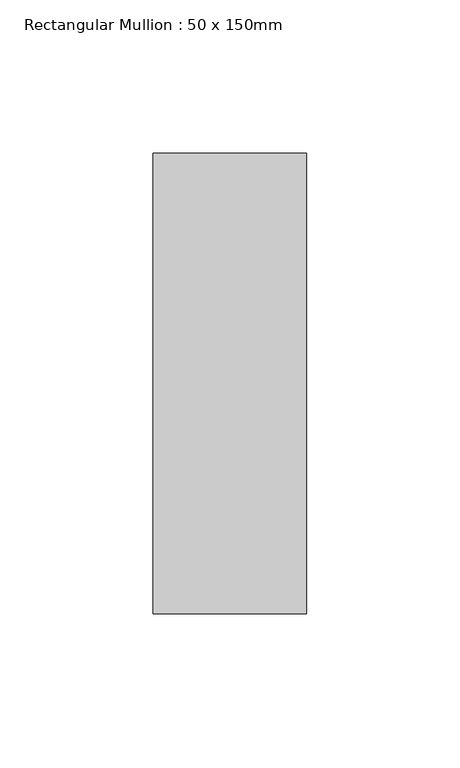
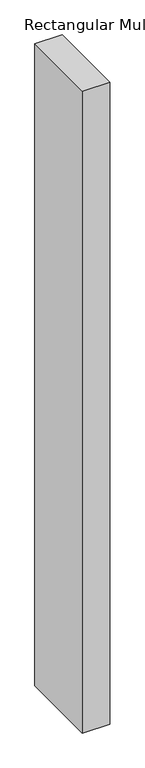
"""IFC4 building model written with IfcOpenShell, lengths in millimetres: member geometry, Rectangular Mullion : 50 x 150mm."""

from ifc_helpers import new_model, si_unit, frame, origin, place, context, project, spatial, polyline, outline, extrude, source, transform, mapped, element, save


def rectangular_mullion_50_x_150mm_49395e3f(model_context):
    return source(origin(), model_context, "Body", "SweptSolid", [
        extrude(outline(polyline([(0.0, 75.0), (0.0, -75.0), (-50.0, -75.0), (-50.0, 75.0), (0.0, 75.0)])), frame((0.0, 0.0, -1240.0000002), z_axis=(0.0, 0.0, 1.0), x_axis=(1.0, 0.0, 0.0)), (0.0, 0.0, 1.0), 1240.0000002),
    ])


if __name__ == "__main__":
    model = new_model("IFC4")
    model_context = context("Model", 3, world=origin())
    ifc_project = project(units=[si_unit("LENGTHUNIT", "METRE", prefix="MILLI")], contexts=[model_context])
    site = spatial("IfcSite", under=ifc_project)
    building = spatial("IfcBuilding", under=site)
    placement = place(None, origin())
    rectangular_mullion_50_x_150mm_shape = rectangular_mullion_50_x_150mm_49395e3f(model_context)
    element("IfcMember", 1, ObjectType="Rectangular Mullion : 50 x 150mm", at=placement, inside=building, context=model_context, shape_type="MappedRepresentation", body=[
        mapped(rectangular_mullion_50_x_150mm_shape, transform((0.0, 0.0, 0.0), x_axis=(1.0, 0.0, 0.0), y_axis=(0.0, 1.0, 0.0), z_axis=(0.0, 0.0, 1.0))),
    ])
    save(model, "model.ifc")

# Revit data of these elements
# Type "Rectangular Mullion : 50 x 150mm"
#   built-in parameter 1007304 = 0.492126 (stored number, unit not read)
#   built-in parameter 1007301 = 0.082021 (stored number, unit not read)
#   built-in parameter 1007300 = 0.082021 (stored number, unit not read)
# Element 1 (IfcMember, "Rectangular Mullion : 50 x 150mm")
#   Materials on its faces: "Aluminium"
# Materials
#   "Aluminium": class "Metal", colour RGB 247 247 247, transparency 0, Description = "Aluminium 6061", Cost = 0
